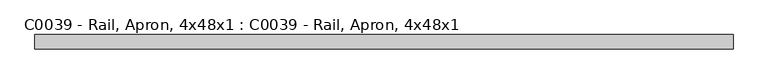
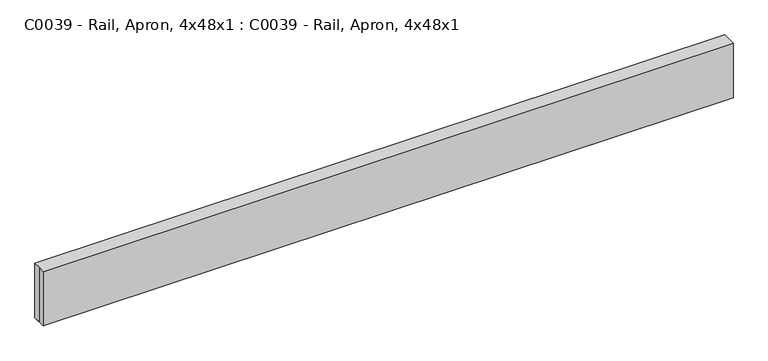
"""IFC4 building model written with IfcOpenShell, lengths in millimetres: proxy geometry, C0039 - Rail, Apron, 4x48x1 : C0039 - Rail, Apron, 4x48x1."""

import ifcopenshell
import ifcopenshell.guid

model = None  # the IFC model being written
_history = None  # IfcOwnerHistory: only IFC2X3 demands one
_inside = {}  # id of a spatial element -> (the spatial element, [elements in it])
_under = {}  # id of a project, library or spatial element -> (it, [spatial elements below it])
_declared = {}  # id of a project -> (the project, [libraries it declares])
_typed = {}  # id of a type object -> (the type object, [elements of that type])
_made_of = {}  # id of a material, layer set ... -> (it, [elements and type objects made of it])


def new_model(schema):
    """Start an empty IFC model of exactly this schema.

    Asked for "IFC4X3", IfcOpenShell would pick the latest addendum, in which some entities
    have other attributes; the version numbers below select the first issue.
    IFC2X3 requires an IfcOwnerHistory on every rooted entity: one is made here for all.
    """
    global model, _history
    if schema == "IFC4X3":
        model = ifcopenshell.file(schema_version=(4, 3, 0, 0))
    else:
        model = ifcopenshell.file(schema=schema)
    _inside.clear()
    _under.clear()
    _declared.clear()
    _typed.clear()
    _made_of.clear()
    _history = None
    if model.schema == "IFC2X3":
        org = make("IfcOrganization", Name="unknown")
        user = make(
            "IfcPersonAndOrganization",
            ThePerson=make("IfcPerson", FamilyName="unknown"),
            TheOrganization=org,
        )
        app = make(
            "IfcApplication",
            ApplicationDeveloper=org,
            Version="unknown",
            ApplicationFullName="unknown",
            ApplicationIdentifier="unknown",
        )
        _history = make(
            "IfcOwnerHistory",
            OwningUser=user,
            OwningApplication=app,
            ChangeAction="ADDED",
            CreationDate=0,
        )
    return model


def make(cls, **values):
    """One entity of the class cls with the attributes given. An attribute that is None is left unset."""
    return model.create_entity(
        cls, **{name: value for name, value in values.items() if value is not None}
    )


def rooted(cls, **values):
    """An entity with a GlobalId (a new one), such as an element, a storey or a relation."""
    return make(cls, GlobalId=ifcopenshell.guid.new(), OwnerHistory=_history, **values)


def si_unit(unit_type, name, prefix=None):
    """IfcSIUnit, for example si_unit("LENGTHUNIT", "METRE", prefix="MILLI")."""
    return make("IfcSIUnit", UnitType=unit_type, Prefix=prefix, Name=name)


def assignment(units):
    """IfcUnitAssignment: the units of a project."""
    return None if units is None else make("IfcUnitAssignment", Units=units)


def point(xyz):
    """IfcCartesianPoint."""
    return None if xyz is None else make("IfcCartesianPoint", Coordinates=xyz)


def direction(xyz):
    """IfcDirection."""
    return None if xyz is None else make("IfcDirection", DirectionRatios=xyz)


def frame(location, z_axis=None, x_axis=None):
    """IfcAxis2Placement3D, a coordinate frame: its origin and axes. An axis left out is left unset."""
    return make(
        "IfcAxis2Placement3D",
        Location=point(location),
        Axis=direction(z_axis),
        RefDirection=direction(x_axis),
    )


def origin():
    """The frame at (0, 0, 0) with its axes left unset."""
    return frame((0.0, 0.0, 0.0))


def origin_with_axes():
    """The frame at (0, 0, 0) with the z axis (0, 0, 1) and the x axis (1, 0, 0) written out."""
    return frame((0.0, 0.0, 0.0), z_axis=(0.0, 0.0, 1.0), x_axis=(1.0, 0.0, 0.0))


def place(relative_to, where):
    """IfcLocalPlacement: puts the frame where relative to a parent placement (None: the world)."""
    return make(
        "IfcLocalPlacement", PlacementRelTo=relative_to, RelativePlacement=where
    )


def context(
    kind, dimensions, precision=None, world=None, true_north=None, identifier=None
):
    """IfcGeometricRepresentationContext, for example the 3D "Model" context."""
    return make(
        "IfcGeometricRepresentationContext",
        ContextIdentifier=identifier,
        ContextType=kind,
        CoordinateSpaceDimension=dimensions,
        Precision=precision,
        WorldCoordinateSystem=world,
        TrueNorth=true_north,
    )


def project(units=None, contexts=None):
    """IfcProject with its units and contexts."""
    return rooted(
        "IfcProject",
        Name="project",
        RepresentationContexts=contexts,
        UnitsInContext=assignment(units),
    )


def spatial(cls, under=None, at=None, **own):
    """A site, building, storey or space (cls), placed at a placement, below another one or the project."""
    s = rooted(cls, ObjectPlacement=at, **own)
    if under is not None:
        _under.setdefault(under.id(), (under, []))[1].append(s)
    return s


def polyline(points):
    """IfcPolyline through the points."""
    return make("IfcPolyline", Points=[point(p) for p in points])


def outline(outer, holes=None, kind="AREA"):
    """IfcArbitraryClosedProfileDef: a profile drawn as a closed curve; with holes, ...WithVoids."""
    if holes is None:
        return make("IfcArbitraryClosedProfileDef", ProfileType=kind, OuterCurve=outer)
    return make(
        "IfcArbitraryProfileDefWithVoids",
        ProfileType=kind,
        OuterCurve=outer,
        InnerCurves=holes,
    )


def extrude(swept, where, along, depth):
    """IfcExtrudedAreaSolid: the profile swept, set in the frame where, extruded along a direction by depth."""
    return make(
        "IfcExtrudedAreaSolid",
        SweptArea=swept,
        Position=where,
        ExtrudedDirection=direction(along),
        Depth=depth,
    )


def shape(context_of_items, identifier, shape_type, items):
    """IfcShapeRepresentation: the items that make up one representation, for example the "Body"."""
    return make(
        "IfcShapeRepresentation",
        ContextOfItems=context_of_items,
        RepresentationIdentifier=identifier,
        RepresentationType=shape_type,
        Items=items,
    )


def source(mapping_origin, context_of_items, identifier, shape_type, items):
    """IfcRepresentationMap: a shape defined once, which mapped items show again and again."""
    return make(
        "IfcRepresentationMap",
        MappingOrigin=mapping_origin,
        MappedRepresentation=shape(context_of_items, identifier, shape_type, items),
    )


def transform(
    local_origin,
    x_axis=None,
    y_axis=None,
    z_axis=None,
    scale=None,
    scale2=None,
    scale3=None,
    uniform=True,
):
    """IfcCartesianTransformationOperator3D, or its non-uniform kind. x_axis, y_axis, z_axis: its Axis1, 2, 3."""
    if uniform:
        return make(
            "IfcCartesianTransformationOperator3D",
            Axis1=direction(x_axis),
            Axis2=direction(y_axis),
            LocalOrigin=point(local_origin),
            Scale=scale,
            Axis3=direction(z_axis),
        )
    return make(
        "IfcCartesianTransformationOperator3DnonUniform",
        Axis1=direction(x_axis),
        Axis2=direction(y_axis),
        LocalOrigin=point(local_origin),
        Scale=scale,
        Axis3=direction(z_axis),
        Scale2=scale2,
        Scale3=scale3,
    )


def mapped(mapping_source, mapping_target):
    """IfcMappedItem: shows the shape of a source again, moved by a transform."""
    return make(
        "IfcMappedItem", MappingSource=mapping_source, MappingTarget=mapping_target
    )


def made_of(thing, what):
    """Note that an element or type object is made of a material, layer set ...; save() writes the relation."""
    if what is not None:
        _made_of.setdefault(what.id(), (what, []))[1].append(thing)
    return thing


def element(
    cls,
    number,
    at=None,
    inside=None,
    cuts=None,
    type_object=None,
    material=None,
    context=None,
    identifier="Body",
    shape_type=None,
    held_by="IfcProductDefinitionShape",
    body=None,
    shapes=None,
    **own,
):
    """One element of the class cls, such as IfcWall. Its Tag is "e" and its number.

    at: its placement. inside: the storey or other place that contains it. cuts: it is an
    opening in that element (IfcRelVoidsElement). A single representation is given by context,
    identifier, shape_type and body (its items); several are given by shapes. held_by: the class
    of the entity that holds the representations. save() writes the other relations.
    """
    e = rooted(cls, Tag="e%d" % number, ObjectPlacement=at, **own)
    if body is not None:
        shapes = [shape(context, identifier, shape_type, body)]
    if shapes is not None:
        e.Representation = make(held_by, Representations=shapes)
    if inside is not None:
        _inside.setdefault(inside.id(), (inside, []))[1].append(e)
    if cuts is not None:
        rooted(
            "IfcRelVoidsElement", RelatingBuildingElement=cuts, RelatedOpeningElement=e
        )
    if type_object is not None:
        _typed.setdefault(type_object.id(), (type_object, []))[1].append(e)
    return made_of(e, material)


def aggregate(whole, parts):
    """IfcRelAggregates: a whole, such as a stair, and the parts it consists of."""
    return rooted("IfcRelAggregates", RelatingObject=whole, RelatedObjects=parts)


def save(model, path):
    """Write the relations noted so far, then the file.

    IfcRelAggregates (storeys below a building ...), IfcRelContainedInSpatialStructure (elements
    in a storey), IfcRelDefinesByType, IfcRelAssociatesMaterial and IfcRelDeclares: one each for
    every whole, place, type object, material and project.
    """
    for whole, parts in _under.values():
        aggregate(whole, parts)
    for where, things in _inside.values():
        rooted(
            "IfcRelContainedInSpatialStructure",
            RelatedElements=things,
            RelatingStructure=where,
        )
    for kind, things in _typed.values():
        rooted("IfcRelDefinesByType", RelatedObjects=things, RelatingType=kind)
    for what, things in _made_of.values():
        rooted("IfcRelAssociatesMaterial", RelatedObjects=things, RelatingMaterial=what)
    for by, libraries in _declared.values():
        rooted("IfcRelDeclares", RelatingContext=by, RelatedDefinitions=libraries)
    model.write(path)


def c0039_rail_apron_4x48x1_c0039_rail_apron_4x48x1_e2c543dd(model_context):
    return source(origin(), model_context, "Body", "SweptSolid", [
        extrude(outline(polyline([(-609.6, 12.7), (609.6, 12.7), (609.6, -12.7), (-609.6, -12.7), (-609.6, 0.0), (-609.6, 12.7)])), origin_with_axes(), (0.0, 0.0, 1.0), 101.6),
        extrude(outline(polyline([(609.6, -12.7), (-609.6, -12.7), (-609.6, 12.7), (609.6, 12.7), (609.6, -12.7)])), origin_with_axes(), (0.0, 0.0, 1.0), 101.6),
    ])


if __name__ == "__main__":
    model = new_model("IFC4")
    model_context = context("Model", 3, world=origin())
    ifc_project = project(units=[si_unit("LENGTHUNIT", "METRE", prefix="MILLI")], contexts=[model_context])
    site = spatial("IfcSite", under=ifc_project)
    building = spatial("IfcBuilding", under=site)
    placement = place(None, origin())
    c0039_rail_apron_4x48x1_c0039_rail_apron_4x48x1_shape = c0039_rail_apron_4x48x1_c0039_rail_apron_4x48x1_e2c543dd(model_context)
    element("IfcBuildingElementProxy", 1, Name="C0039 - Rail, Apron, 4x48x1 : C0039 - Rail, Apron, 4x48x1", ObjectType="C0039 - Rail, Apron, 4x48x1 : C0039 - Rail, Apron, 4x48x1", at=placement, inside=building, context=model_context, shape_type="MappedRepresentation", body=[
        mapped(c0039_rail_apron_4x48x1_c0039_rail_apron_4x48x1_shape, transform((0.0, 0.0, 0.0), x_axis=(1.0, 0.0, 0.0), y_axis=(0.0, 1.0, 0.0), z_axis=(0.0, 0.0, 1.0))),
    ])
    save(model, "model.ifc")

# Revit data of these elements
# Type "C0039 - Rail, Apron, 4x48x1 : C0039 - Rail, Apron, 4x48x1"
#   Watts2 = "0"
#   Watts1 = "0"
#   Unit_Issue = "EA"
#   UTIL_6_Misc = "-"
#   UTIL_5_NonMedGas = "-"
#   UTIL_4_MiscGas = "-"
#   UTIL_3_MedGas = "-"
#   UTIL_2_Elec = "-"
#   UTIL_1_WaterDrain = "-"
#   Nomenclature = "Rail, Apron, 4x48x1"
#   NSN = "6530"
#   Location [instance default] = ""
#   JSN = "C0039"
#   Fund_Source_VA = "-"
#   Fund_Source_Navy = "-"
#   Fund_Source_Army = "-"
#   Fund_Source_AF = "-"
#   ELEC_Volts2 = "0"
#   ELEC_Volts1 = "0"
#   ELEC_Phase2 = "0"
#   ELEC_Phase1 = "0"
#   ELEC_HertzSwitch = "0"
#   ELEC_HertzDependent = "0"
#   ELEC_Hertz = "0"
#   ELEC_Amps2 = "0"
#   ELEC_Amps1 = "0"
#   DetailDescription = "Apron rail. Also referred to as an apron front, apron panel, or knee space rail. Used to close in front knee space area and/or provide work surface support between two base cabinets or a base cabinet and wall. Apron rails should be ordered in pairs to provide both front and rear work surface support."
#   CAT_VA = "A"
#   CAT_Navy = "A"
#   CAT_IHS = "-"
#   CAT_Army = "A"
#   CAT_AF = "A"
#   BTUperhour = "0"
#   Weight_IP = 14
#   DIM_Width_IP = 4' - 0"
#   DIM_Height_IP = 0' - 4"
#   DIM_Depth_IP = 0' - 1"
#   Top Panel Material = none
#   Toe Panel Material = none
#   Side Panel Material = none
#   Shelf Panel Material = none
#   Drawer Front Material = none
#   Door Panel Material = none
#   Back Panel Material = none
#   Assembly Code = ""
# Element 1 (IfcBuildingElementProxy, "C0039 - Rail, Apron, 4x48x1 : C0039 - Rail, Apron, 4x48x1")
#   Materials on its faces: "EquipSpace"
# Materials
#   "EquipSpace": class "Unassigned", colour RGB 221 217 195, transparency 0.5
